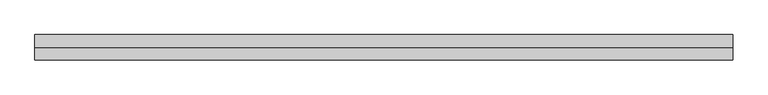
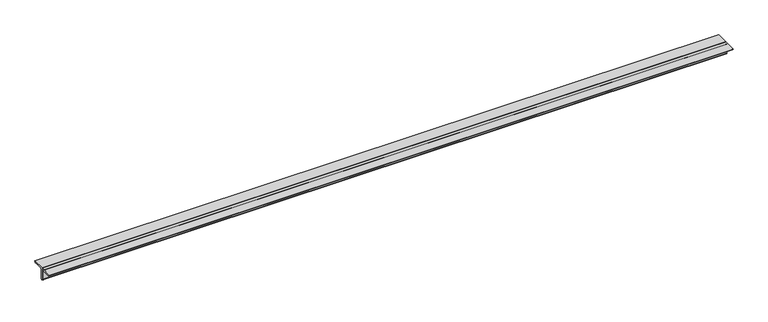
"""IFC4 building model written with IfcOpenShell, lengths in millimetres: member geometry, Steel Framing_2Ls_KS : H_SB_AR_S02_2Ls-100x100x10_VBR1."""

from ifc_helpers import new_model, si_unit, point, frame, frame_2d, origin, place, context, project, spatial, polyline, circle_curve, trimmed, segment, composite_curve, outline, extrude, source, transform, mapped, element, save


def member_3b71fc5b(model_context):
    return source(origin(), model_context, "Body", "SweptSolid", [
        extrude(outline(composite_curve([segment(polyline([(0.0, 28.2), (100.0, 28.2)]), True, "CONTINUOUS"), segment(trimmed(circle_curve(frame_2d((90.0, 28.2)), 10.0), [point((100.0, 28.2))], [point((90.0, 18.2))], False, "CARTESIAN"), True, "CONTINUOUS"), segment(polyline([(90.0, 18.2), (20.0, 18.2)]), True, "CONTINUOUS"), segment(trimmed(circle_curve(frame_2d((20.0, 8.2)), 10.0), [point((20.0, 18.2))], [point((10.0, 8.2))], True, "CARTESIAN"), True, "CONTINUOUS"), segment(polyline([(10.0, 8.2), (10.0, -61.8)]), True, "CONTINUOUS"), segment(trimmed(circle_curve(frame_2d((0.0, -61.8)), 10.0), [point((10.0, -61.8))], [point((0.0, -71.8))], False, "CARTESIAN"), True, "CONTINUOUS"), segment(polyline([(0.0, -71.8), (0.0, 28.2)]), True, "CONTINUOUS")], self_intersect=False)), frame((-2813.1509912, 0.0, 0.0), z_axis=(1.0, 0.0, 0.0), x_axis=(0.0, 1.0, 0.0)), (0.0, 0.0, 1.0), 5533.812112),
        extrude(outline(composite_curve([segment(polyline([(0.0, 28.2), (0.0, -71.8)]), True, "CONTINUOUS"), segment(trimmed(circle_curve(frame_2d((0.0, -61.8)), 10.0), [point((0.0, -71.8))], [point((-10.0, -61.8))], False, "CARTESIAN"), True, "CONTINUOUS"), segment(polyline([(-10.0, -61.8), (-10.0, 8.2)]), True, "CONTINUOUS"), segment(trimmed(circle_curve(frame_2d((-20.0, 8.2)), 10.0), [point((-10.0, 8.2))], [point((-20.0, 18.2))], True, "CARTESIAN"), True, "CONTINUOUS"), segment(polyline([(-20.0, 18.2), (-90.0, 18.2)]), True, "CONTINUOUS"), segment(trimmed(circle_curve(frame_2d((-90.0, 28.2)), 10.0), [point((-90.0, 18.2))], [point((-100.0, 28.2))], False, "CARTESIAN"), True, "CONTINUOUS"), segment(polyline([(-100.0, 28.2), (0.0, 28.2)]), True, "CONTINUOUS")], self_intersect=False)), frame((-2813.1509912, 0.0, 0.0), z_axis=(1.0, 0.0, 0.0), x_axis=(0.0, 1.0, 0.0)), (0.0, 0.0, 1.0), 5533.812112),
    ])


if __name__ == "__main__":
    model = new_model("IFC4")
    model_context = context("Model", 3, world=origin())
    ifc_project = project(units=[si_unit("LENGTHUNIT", "METRE", prefix="MILLI")], contexts=[model_context])
    site = spatial("IfcSite", under=ifc_project)
    building = spatial("IfcBuilding", under=site)
    placement = place(None, origin())
    member_shape = member_3b71fc5b(model_context)
    element("IfcMember", 1, ObjectType="Steel Framing_2Ls_KS : H_SB_AR_S02_2Ls-100x100x10_VBR1", at=placement, inside=building, context=model_context, shape_type="MappedRepresentation", body=[
        mapped(member_shape, transform((0.0, 0.0, 0.0), x_axis=(1.0, 0.0, 0.0), y_axis=(0.0, 1.0, 0.0), z_axis=(0.0, 0.0, 1.0))),
    ])
    save(model, "model.ifc")

# Revit data of these elements
# Type "Steel Framing_2Ls_KS : H_SB_AR_S02_2Ls-100x100x10_VBR1"
#   Type Comments = "MAIN"
#   Type Mark = "VBR1"
#   H_SectionID = "2Ls-100x100x10"
#   Assembly Code = "B10"
#   Legs = "LLBB"
#   H_Ratio for Additional Steel Plate = 0.2
#   W = 0
#   Perimeter = 0.80 m²/m
#   Nominal Weight = 29.80 kgf/m
#   Length [instance default] = 1524 mm
#   Space = 0 mm
#   b = 100 mm
#   d = 100 mm
#   t = 10 mm
#   y = 28.2 mm
#   A = 0.0038 m²
#   Structural Material [instance default] = Steel, 45-345
# Element 1 (IfcMember, "Steel Framing_2Ls_KS : H_SB_AR_S02_2Ls-100x100x10_VBR1")
#   Materials on its faces: "Steel, 45-345"
# Materials
#   "Steel, 45-345": class "Metal", colour RGB 189 187 185, transparency 0, Description = "Steel 345 MPa", Cost = 0
